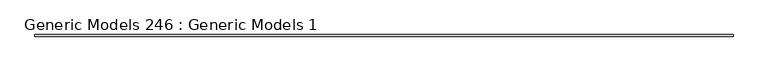
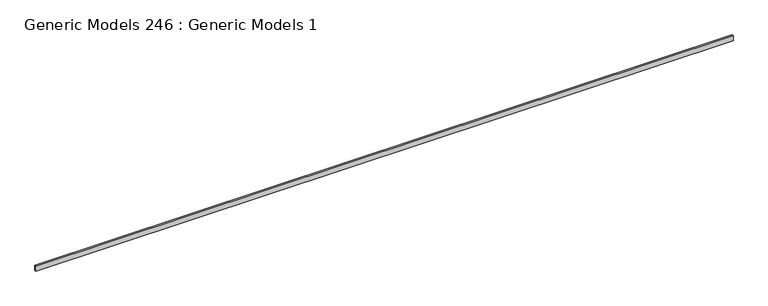
"""IFC4 building model written with IfcOpenShell, lengths in millimetres: proxy geometry, Generic Models 246 : Generic Models 1."""

from ifc_helpers import new_model, si_unit, frame, origin, place, context, project, spatial, polyline, outline, extrude, source, transform, mapped, element, save


def generic_models_246_generic_models_1_2de35281(model_context):
    return source(origin(), model_context, "Body", "SweptSolid", [
        extrude(outline(polyline([(-5248.1628079, -20141.8223745), (-5248.1628079, -20097.3723745), (13801.8371921, -20097.3723745), (13801.8371921, -20141.8223745), (-5248.1628079, -20141.8223745)])), frame((0.0, 0.0, 126814.0999329), z_axis=(0.0, 0.0, 1.0), x_axis=(1.0, 0.0, 0.0)), (0.0, 0.0, 1.0), 139.7),
    ])


if __name__ == "__main__":
    model = new_model("IFC4")
    model_context = context("Model", 3, world=origin())
    ifc_project = project(units=[si_unit("LENGTHUNIT", "METRE", prefix="MILLI")], contexts=[model_context])
    site = spatial("IfcSite", under=ifc_project)
    building = spatial("IfcBuilding", under=site)
    placement = place(None, origin())
    generic_models_246_generic_models_1_shape = generic_models_246_generic_models_1_2de35281(model_context)
    element("IfcBuildingElementProxy", 1, Name="Generic Models 246 : Generic Models 1", ObjectType="Generic Models 246 : Generic Models 1", at=placement, inside=building, context=model_context, shape_type="MappedRepresentation", body=[
        mapped(generic_models_246_generic_models_1_shape, transform((0.0, 0.0, 0.0), x_axis=(1.0, 0.0, 0.0), y_axis=(0.0, 1.0, 0.0), z_axis=(0.0, 0.0, 1.0))),
    ])
    save(model, "model.ifc")

# Revit data of these elements
# Element 1 (IfcBuildingElementProxy, "Generic Models 246 : Generic Models 1")
#   Materials on its faces: "_STRUCTURAL MEMBER (SEE STRUCT. DWGS)"
# Materials
#   "_STRUCTURAL MEMBER (SEE STRUCT. DWGS)": class "Generic", colour RGB 209 182 141, transparency 0, Cost = 0
